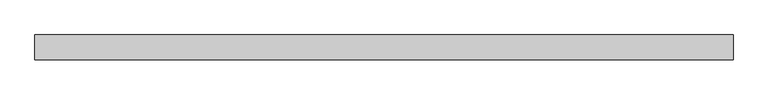
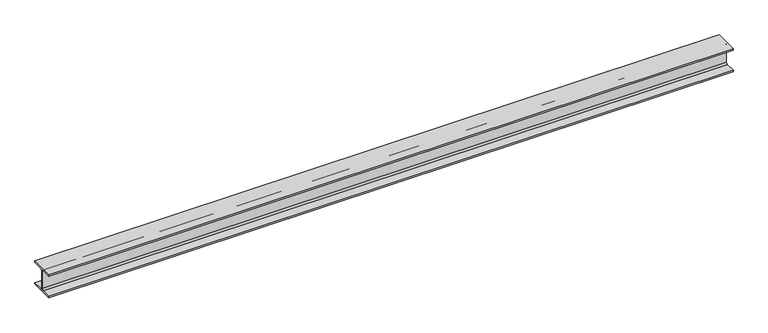
"""IFC4 building model written with IfcOpenShell, lengths in millimetres: beam geometry, 0912_Steel Framing_H-KSD3502 : H_SB_ASB_H-200x200x8x12."""

from ifc_helpers import new_model, si_unit, point, frame, frame_2d, origin, place, context, project, spatial, polyline, circle_curve, trimmed, segment, composite_curve, outline, extrude, source, transform, mapped, element, save


def beam_35a77e60(model_context):
    return source(origin(), model_context, "Body", "SweptSolid", [
        extrude(outline(composite_curve([segment(polyline([(100.0, -88.0), (100.0, -100.0), (-100.0, -100.0), (-100.0, -88.0), (-17.0, -88.0)]), True, "CONTINUOUS"), segment(trimmed(circle_curve(frame_2d((-17.0, -75.0)), 13.0), [point((-17.0, -88.0))], [point((-4.0, -75.0))], True, "CARTESIAN"), True, "CONTINUOUS"), segment(polyline([(-4.0, -75.0), (-4.0, 75.0)]), True, "CONTINUOUS"), segment(trimmed(circle_curve(frame_2d((-17.0, 75.0)), 13.0), [point((-4.0, 75.0))], [point((-17.0, 88.0))], True, "CARTESIAN"), True, "CONTINUOUS"), segment(polyline([(-17.0, 88.0), (-100.0, 88.0), (-100.0, 100.0), (100.0, 100.0), (100.0, 88.0), (17.0, 88.0)]), True, "CONTINUOUS"), segment(trimmed(circle_curve(frame_2d((17.0, 75.0)), 13.0), [point((17.0, 88.0))], [point((4.0, 75.0))], True, "CARTESIAN"), True, "CONTINUOUS"), segment(polyline([(4.0, 75.0), (4.0, -75.0)]), True, "CONTINUOUS"), segment(trimmed(circle_curve(frame_2d((17.0, -75.0)), 13.0), [point((4.0, -75.0))], [point((17.0, -88.0))], True, "CARTESIAN"), True, "CONTINUOUS"), segment(polyline([(17.0, -88.0), (100.0, -88.0)]), True, "CONTINUOUS")], self_intersect=False)), frame((-2836.3595741, 0.0, 0.0), z_axis=(1.0, 0.0, 0.0), x_axis=(0.0, 1.0, 0.0)), (0.0, 0.0, 1.0), 5644.3797083),
    ])


if __name__ == "__main__":
    model = new_model("IFC4")
    model_context = context("Model", 3, world=origin())
    ifc_project = project(units=[si_unit("LENGTHUNIT", "METRE", prefix="MILLI")], contexts=[model_context])
    site = spatial("IfcSite", under=ifc_project)
    building = spatial("IfcBuilding", under=site)
    placement = place(None, origin())
    beam_shape = beam_35a77e60(model_context)
    element("IfcBeam", 1, ObjectType="0912_Steel Framing_H-KSD3502 : H_SB_ASB_H-200x200x8x12", at=placement, inside=building, context=model_context, shape_type="MappedRepresentation", body=[
        mapped(beam_shape, transform((0.0, 0.0, 0.0), x_axis=(1.0, 0.0, 0.0), y_axis=(0.0, 1.0, 0.0), z_axis=(0.0, 0.0, 1.0))),
    ])
    save(model, "model.ifc")

# Revit data of these elements
# Type "0912_Steel Framing_H-KSD3502 : H_SB_ASB_H-200x200x8x12"
#   H_WM Code_1 = "S01AA002-00001 | Main Steel Structure Fabrication Work | Shelter/Building | Medium Steel - Standard (90KG/M>Weight≥30KG/M) | Material: (   )"
#   H_WM Code_2 = "S03AA028-00001 | Main Steel Structure Erection Work | Shelter/Building | Medium Steel (90KG/M>Weight≥30KG/M) | Material: (   )"
#   H_WM Code_3 = "S01AA010-00001 | Main Steel Structure Fabrication Work | Shelter/Building | Steel Painting/Coating | for Non-Fireproofed Steel Surface, Surface Preparation, Primer, Second & Final Coat | Material: (   )"
#   H_Q'ty Cal Type Tag = "SB-Q2"
#   Width = 20.0 cm
#   Web Thickness = 0.8 cm
#   Web Fillet = 1.3 cm
#   Warping Constant = 141000.0 cm⁶
#   W = 0
#   Torsional Moment of Inertia = 26.2485 cm⁴
#   Section Area = 63.53 cm²
#   Plastic Modulus weak axis = 244.0 cm³
#   Plastic Modulus strong axis = 525.0 cm³
#   Perimeter = 1.16 m²/m
#   Nominal Weight = 49.90 kgf/m
#   Moment of Inertia weak axis = 1600.00 cm⁴
#   Moment of Inertia strong axis = 4720.00 cm⁴
#   Height = 20.0 cm
#   Flange Thickness = 1.2 cm
#   Elastic Modulus weak axis = 160.0 cm³
#   Elastic Modulus strong axis = 472.0 cm³
#   Centroid Vertical = 10.0 cm
#   Centroid Horizontal = 10.0 cm
#   Ix = 47200000
#   Length [instance default] = 1.5240 m
#   Zx = 525000
#   b = 0.2000 m
#   h = 0.2000 m
#   r = 0.0130 m
#   s = 0.0080 m
#   t = 0.0120 m
#   A = 0.006353 m²
#   Structural Material [instance default] = Steel, 45-345
#   Assembly Code = ""
# Element 1 (IfcBeam, "0912_Steel Framing_H-KSD3502 : H_SB_ASB_H-200x200x8x12")
#   Structural Material = none
# Materials
#   "Steel, 45-345": class "Metal", colour RGB 189 187 185, transparency 0, Description = "Steel 345 MPa", Cost = 0
